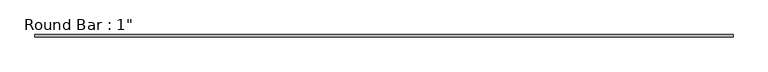
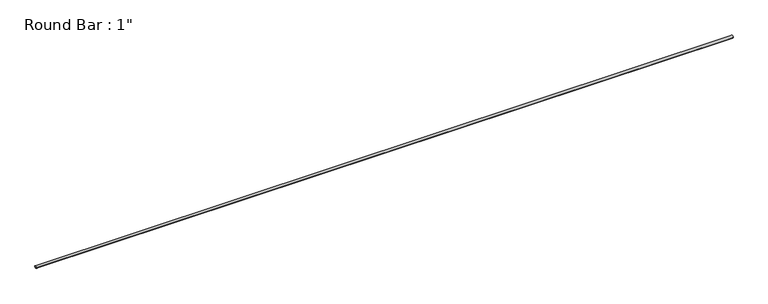
"""IFC4 building model written with IfcOpenShell, lengths in millimetres: member geometry."""

import ifcopenshell
import ifcopenshell.guid

model = None  # the IFC model being written
_history = None  # IfcOwnerHistory: only IFC2X3 demands one
_inside = {}  # id of a spatial element -> (the spatial element, [elements in it])
_under = {}  # id of a project, library or spatial element -> (it, [spatial elements below it])
_declared = {}  # id of a project -> (the project, [libraries it declares])
_typed = {}  # id of a type object -> (the type object, [elements of that type])
_made_of = {}  # id of a material, layer set ... -> (it, [elements and type objects made of it])


def new_model(schema):
    """Start an empty IFC model of exactly this schema.

    Asked for "IFC4X3", IfcOpenShell would pick the latest addendum, in which some entities
    have other attributes; the version numbers below select the first issue.
    IFC2X3 requires an IfcOwnerHistory on every rooted entity: one is made here for all.
    """
    global model, _history
    if schema == "IFC4X3":
        model = ifcopenshell.file(schema_version=(4, 3, 0, 0))
    else:
        model = ifcopenshell.file(schema=schema)
    _inside.clear()
    _under.clear()
    _declared.clear()
    _typed.clear()
    _made_of.clear()
    _history = None
    if model.schema == "IFC2X3":
        org = make("IfcOrganization", Name="unknown")
        user = make(
            "IfcPersonAndOrganization",
            ThePerson=make("IfcPerson", FamilyName="unknown"),
            TheOrganization=org,
        )
        app = make(
            "IfcApplication",
            ApplicationDeveloper=org,
            Version="unknown",
            ApplicationFullName="unknown",
            ApplicationIdentifier="unknown",
        )
        _history = make(
            "IfcOwnerHistory",
            OwningUser=user,
            OwningApplication=app,
            ChangeAction="ADDED",
            CreationDate=0,
        )
    return model


def make(cls, **values):
    """One entity of the class cls with the attributes given. An attribute that is None is left unset."""
    return model.create_entity(
        cls, **{name: value for name, value in values.items() if value is not None}
    )


def rooted(cls, **values):
    """An entity with a GlobalId (a new one), such as an element, a storey or a relation."""
    return make(cls, GlobalId=ifcopenshell.guid.new(), OwnerHistory=_history, **values)


def si_unit(unit_type, name, prefix=None):
    """IfcSIUnit, for example si_unit("LENGTHUNIT", "METRE", prefix="MILLI")."""
    return make("IfcSIUnit", UnitType=unit_type, Prefix=prefix, Name=name)


def assignment(units):
    """IfcUnitAssignment: the units of a project."""
    return None if units is None else make("IfcUnitAssignment", Units=units)


def point(xyz):
    """IfcCartesianPoint."""
    return None if xyz is None else make("IfcCartesianPoint", Coordinates=xyz)


def direction(xyz):
    """IfcDirection."""
    return None if xyz is None else make("IfcDirection", DirectionRatios=xyz)


def frame(location, z_axis=None, x_axis=None):
    """IfcAxis2Placement3D, a coordinate frame: its origin and axes. An axis left out is left unset."""
    return make(
        "IfcAxis2Placement3D",
        Location=point(location),
        Axis=direction(z_axis),
        RefDirection=direction(x_axis),
    )


def frame_2d(location, x_axis=None):
    """IfcAxis2Placement2D, a coordinate frame in the plane: its origin and x axis."""
    return make(
        "IfcAxis2Placement2D", Location=point(location), RefDirection=direction(x_axis)
    )


def origin():
    """The frame at (0, 0, 0) with its axes left unset."""
    return frame((0.0, 0.0, 0.0))


def origin_2d():
    """The frame at (0, 0) in the plane with its x axis left unset."""
    return frame_2d((0.0, 0.0))


def place(relative_to, where):
    """IfcLocalPlacement: puts the frame where relative to a parent placement (None: the world)."""
    return make(
        "IfcLocalPlacement", PlacementRelTo=relative_to, RelativePlacement=where
    )


def context(
    kind, dimensions, precision=None, world=None, true_north=None, identifier=None
):
    """IfcGeometricRepresentationContext, for example the 3D "Model" context."""
    return make(
        "IfcGeometricRepresentationContext",
        ContextIdentifier=identifier,
        ContextType=kind,
        CoordinateSpaceDimension=dimensions,
        Precision=precision,
        WorldCoordinateSystem=world,
        TrueNorth=true_north,
    )


def project(units=None, contexts=None):
    """IfcProject with its units and contexts."""
    return rooted(
        "IfcProject",
        Name="project",
        RepresentationContexts=contexts,
        UnitsInContext=assignment(units),
    )


def spatial(cls, under=None, at=None, **own):
    """A site, building, storey or space (cls), placed at a placement, below another one or the project."""
    s = rooted(cls, ObjectPlacement=at, **own)
    if under is not None:
        _under.setdefault(under.id(), (under, []))[1].append(s)
    return s


def circle_curve(where, radius):
    """IfcCircle in the frame where."""
    return make("IfcCircle", Position=where, Radius=radius)


def trimmed(basis, trim1, trim2, sense, master):
    """IfcTrimmedCurve: the piece of a basis curve between two trims."""
    return make(
        "IfcTrimmedCurve",
        BasisCurve=basis,
        Trim1=trim1,
        Trim2=trim2,
        SenseAgreement=sense,
        MasterRepresentation=master,
    )


def segment(curve, same_sense, transition):
    """IfcCompositeCurveSegment."""
    return make(
        "IfcCompositeCurveSegment",
        Transition=transition,
        SameSense=same_sense,
        ParentCurve=curve,
    )


def composite_curve(segments, self_intersect=None):
    """IfcCompositeCurve: segments joined end to end."""
    return make("IfcCompositeCurve", Segments=segments, SelfIntersect=self_intersect)


def outline(outer, holes=None, kind="AREA"):
    """IfcArbitraryClosedProfileDef: a profile drawn as a closed curve; with holes, ...WithVoids."""
    if holes is None:
        return make("IfcArbitraryClosedProfileDef", ProfileType=kind, OuterCurve=outer)
    return make(
        "IfcArbitraryProfileDefWithVoids",
        ProfileType=kind,
        OuterCurve=outer,
        InnerCurves=holes,
    )


def extrude(swept, where, along, depth):
    """IfcExtrudedAreaSolid: the profile swept, set in the frame where, extruded along a direction by depth."""
    return make(
        "IfcExtrudedAreaSolid",
        SweptArea=swept,
        Position=where,
        ExtrudedDirection=direction(along),
        Depth=depth,
    )


def shape(context_of_items, identifier, shape_type, items):
    """IfcShapeRepresentation: the items that make up one representation, for example the "Body"."""
    return make(
        "IfcShapeRepresentation",
        ContextOfItems=context_of_items,
        RepresentationIdentifier=identifier,
        RepresentationType=shape_type,
        Items=items,
    )


def source(mapping_origin, context_of_items, identifier, shape_type, items):
    """IfcRepresentationMap: a shape defined once, which mapped items show again and again."""
    return make(
        "IfcRepresentationMap",
        MappingOrigin=mapping_origin,
        MappedRepresentation=shape(context_of_items, identifier, shape_type, items),
    )


def transform(
    local_origin,
    x_axis=None,
    y_axis=None,
    z_axis=None,
    scale=None,
    scale2=None,
    scale3=None,
    uniform=True,
):
    """IfcCartesianTransformationOperator3D, or its non-uniform kind. x_axis, y_axis, z_axis: its Axis1, 2, 3."""
    if uniform:
        return make(
            "IfcCartesianTransformationOperator3D",
            Axis1=direction(x_axis),
            Axis2=direction(y_axis),
            LocalOrigin=point(local_origin),
            Scale=scale,
            Axis3=direction(z_axis),
        )
    return make(
        "IfcCartesianTransformationOperator3DnonUniform",
        Axis1=direction(x_axis),
        Axis2=direction(y_axis),
        LocalOrigin=point(local_origin),
        Scale=scale,
        Axis3=direction(z_axis),
        Scale2=scale2,
        Scale3=scale3,
    )


def mapped(mapping_source, mapping_target):
    """IfcMappedItem: shows the shape of a source again, moved by a transform."""
    return make(
        "IfcMappedItem", MappingSource=mapping_source, MappingTarget=mapping_target
    )


def made_of(thing, what):
    """Note that an element or type object is made of a material, layer set ...; save() writes the relation."""
    if what is not None:
        _made_of.setdefault(what.id(), (what, []))[1].append(thing)
    return thing


def element(
    cls,
    number,
    at=None,
    inside=None,
    cuts=None,
    type_object=None,
    material=None,
    context=None,
    identifier="Body",
    shape_type=None,
    held_by="IfcProductDefinitionShape",
    body=None,
    shapes=None,
    **own,
):
    """One element of the class cls, such as IfcWall. Its Tag is "e" and its number.

    at: its placement. inside: the storey or other place that contains it. cuts: it is an
    opening in that element (IfcRelVoidsElement). A single representation is given by context,
    identifier, shape_type and body (its items); several are given by shapes. held_by: the class
    of the entity that holds the representations. save() writes the other relations.
    """
    e = rooted(cls, Tag="e%d" % number, ObjectPlacement=at, **own)
    if body is not None:
        shapes = [shape(context, identifier, shape_type, body)]
    if shapes is not None:
        e.Representation = make(held_by, Representations=shapes)
    if inside is not None:
        _inside.setdefault(inside.id(), (inside, []))[1].append(e)
    if cuts is not None:
        rooted(
            "IfcRelVoidsElement", RelatingBuildingElement=cuts, RelatedOpeningElement=e
        )
    if type_object is not None:
        _typed.setdefault(type_object.id(), (type_object, []))[1].append(e)
    return made_of(e, material)


def aggregate(whole, parts):
    """IfcRelAggregates: a whole, such as a stair, and the parts it consists of."""
    return rooted("IfcRelAggregates", RelatingObject=whole, RelatedObjects=parts)


def save(model, path):
    """Write the relations noted so far, then the file.

    IfcRelAggregates (storeys below a building ...), IfcRelContainedInSpatialStructure (elements
    in a storey), IfcRelDefinesByType, IfcRelAssociatesMaterial and IfcRelDeclares: one each for
    every whole, place, type object, material and project.
    """
    for whole, parts in _under.values():
        aggregate(whole, parts)
    for where, things in _inside.values():
        rooted(
            "IfcRelContainedInSpatialStructure",
            RelatedElements=things,
            RelatingStructure=where,
        )
    for kind, things in _typed.values():
        rooted("IfcRelDefinesByType", RelatedObjects=things, RelatingType=kind)
    for what, things in _made_of.values():
        rooted("IfcRelAssociatesMaterial", RelatedObjects=things, RelatingMaterial=what)
    for by, libraries in _declared.values():
        rooted("IfcRelDeclares", RelatingContext=by, RelatedDefinitions=libraries)
    model.write(path)


def member_b3c834a1(model_context):
    return source(origin(), model_context, "Body", "SweptSolid", [
        extrude(outline(composite_curve([segment(trimmed(circle_curve(origin_2d(), 12.7), [point((12.7, 0.0))], [point((-12.7, 0.0))], False, "CARTESIAN"), True, "CONTINUOUS"), segment(trimmed(circle_curve(origin_2d(), 12.7), [point((-12.7, 0.0))], [point((12.7, 0.0))], False, "CARTESIAN"), True, "CONTINUOUS")], self_intersect=False)), frame((-3531.1537482, 0.0, 0.0), z_axis=(1.0, 0.0, 0.0), x_axis=(0.0, 1.0, 0.0)), (0.0, 0.0, 1.0), 7062.3074965),
    ])


if __name__ == "__main__":
    model = new_model("IFC4")
    model_context = context("Model", 3, world=origin())
    ifc_project = project(units=[si_unit("LENGTHUNIT", "METRE", prefix="MILLI")], contexts=[model_context])
    site = spatial("IfcSite", under=ifc_project)
    building = spatial("IfcBuilding", under=site)
    placement = place(None, origin())
    member_shape = member_b3c834a1(model_context)
    element("IfcMember", 1, ObjectType="Round Bar : 1\"", at=placement, inside=building, context=model_context, shape_type="MappedRepresentation", body=[
        mapped(member_shape, transform((0.0, 0.0, 0.0), x_axis=(1.0, 0.0, 0.0), y_axis=(0.0, 1.0, 0.0), z_axis=(0.0, 0.0, 1.0))),
    ])
    save(model, "model.ifc")

# Revit data of these elements
# Type "Round Bar : 1\""
#   Assembly Code = "B10"
#   W = 0
#   Start Extension Calculation [instance default] = 10' - 0"
#   Start Extension [instance default] = -0' - 0 1/2"
#   End Extension Calculation [instance default] = 10' - 0"
#   End Extension [instance default] = -0' - 0 1/2"
#   Length [instance default] = 5' - 0"
#   d = 0' - 1"
#   A = 0 SF
#   Structural Material [instance default] = Metal - Steel - ASTM A36
# Element 1 (IfcMember, "Round Bar : 1\"")
#   Materials on its faces: "Metal - Steel - ASTM A36"
# Materials
#   "Metal - Steel - ASTM A36": class "Metal", colour RGB 199 199 199, transparency 0
